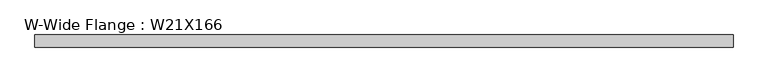
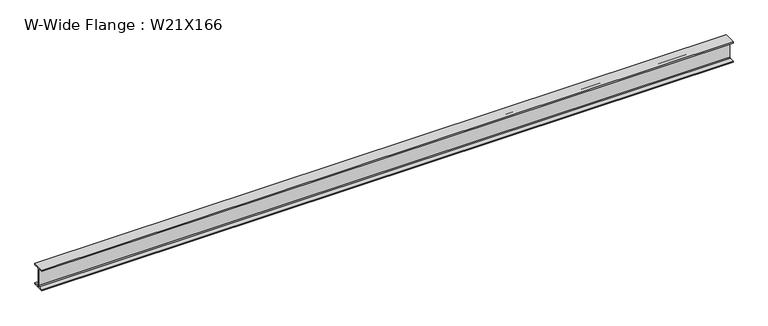
"""IFC4 building model written with IfcOpenShell, lengths in millimetres: beam geometry, W-Wide Flange : W21X166."""

from ifc_helpers import new_model, si_unit, point, frame, frame_2d, origin, place, context, project, spatial, polyline, circle_curve, trimmed, segment, composite_curve, outline, extrude, source, transform, mapped, element, save


def w_wide_flange_w21x166_c8885ad3(model_context):
    return source(origin(), model_context, "Body", "SweptSolid", [
        extrude(outline(composite_curve([segment(polyline([(157.48, -251.206), (157.48, -285.75), (-157.48, -285.75), (-157.48, -251.206), (-32.131, -251.206)]), True, "CONTINUOUS"), segment(trimmed(circle_curve(frame_2d((-32.131, -228.6)), 22.606), [point((-32.131, -251.206))], [point((-9.525, -228.6))], True, "CARTESIAN"), True, "CONTINUOUS"), segment(polyline([(-9.525, -228.6), (-9.525, 228.6)]), True, "CONTINUOUS"), segment(trimmed(circle_curve(frame_2d((-32.131, 228.6)), 22.606), [point((-9.525, 228.6))], [point((-32.131, 251.206))], True, "CARTESIAN"), True, "CONTINUOUS"), segment(polyline([(-32.131, 251.206), (-157.48, 251.206), (-157.48, 285.75), (157.48, 285.75), (157.48, 251.206), (32.131, 251.206)]), True, "CONTINUOUS"), segment(trimmed(circle_curve(frame_2d((32.131, 228.6)), 22.606), [point((32.131, 251.206))], [point((9.525, 228.6))], True, "CARTESIAN"), True, "CONTINUOUS"), segment(polyline([(9.525, 228.6), (9.525, -228.6)]), True, "CONTINUOUS"), segment(trimmed(circle_curve(frame_2d((32.131, -228.6)), 22.606), [point((9.525, -228.6))], [point((32.131, -251.206))], True, "CARTESIAN"), True, "CONTINUOUS"), segment(polyline([(32.131, -251.206), (157.48, -251.206)]), True, "CONTINUOUS")], self_intersect=False)), frame((-9128.1346451, 0.0, 0.0), z_axis=(1.0, 0.0, 0.0), x_axis=(0.0, 1.0, 0.0)), (0.0, 0.0, 1.0), 18150.0379668),
    ])


if __name__ == "__main__":
    model = new_model("IFC4")
    model_context = context("Model", 3, world=origin())
    ifc_project = project(units=[si_unit("LENGTHUNIT", "METRE", prefix="MILLI")], contexts=[model_context])
    site = spatial("IfcSite", under=ifc_project)
    building = spatial("IfcBuilding", under=site)
    placement = place(None, origin())
    w_wide_flange_w21x166_shape = w_wide_flange_w21x166_c8885ad3(model_context)
    element("IfcBeam", 1, ObjectType="W-Wide Flange : W21X166", at=placement, inside=building, context=model_context, shape_type="MappedRepresentation", body=[
        mapped(w_wide_flange_w21x166_shape, transform((0.0, 0.0, 0.0), x_axis=(1.0, 0.0, 0.0), y_axis=(0.0, 1.0, 0.0), z_axis=(0.0, 0.0, 1.0))),
    ])
    save(model, "model.ifc")

# Revit data of these elements
# Type "W-Wide Flange : W21X166"
#   Assembly Code = "B10"
#   W = 166
#   Length [instance default] = 5' - 0"
#   bf = 1' - 0.4"
#   d = 1' - 10 1/2"
#   k = 0' - 2 1/4"
#   k2 = 0' - 0.89"
#   tf = 0' - 1.36"
#   tw = 0' - 0 3/4"
#   A = 0.338889 SF
#   Structural Material [instance default] = Steel ASTM A992
# Element 1 (IfcBeam, "W-Wide Flange : W21X166")
#   Structural Material = Steel
#   Materials on its faces: "Steel"
# Materials
#   "Steel ASTM A992": class "Metal", colour RGB 199 199 199, transparency 0, Description = "Structural steel 50ksi", Cost = 0
#   "Steel": class "Metal", colour RGB 118 118 114, transparency 0, Description = "Steel, mill finish", Cost = 0
